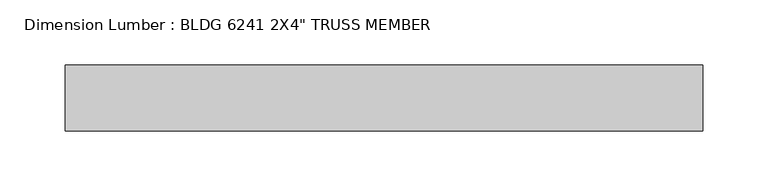
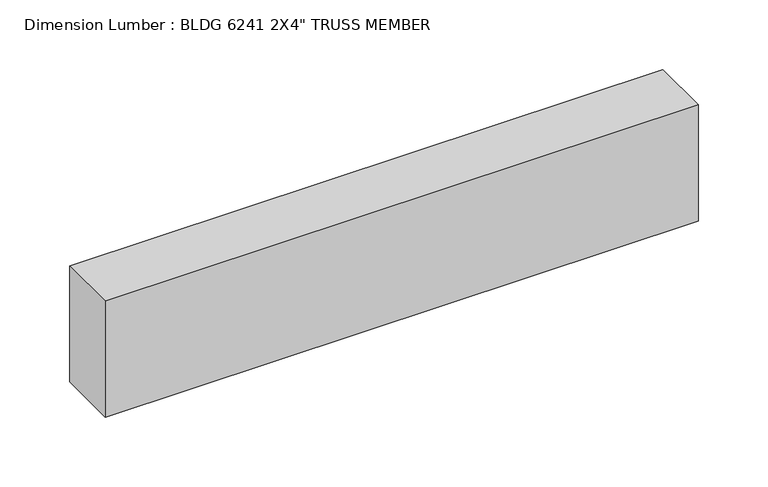
"""IFC4 building model written with IfcOpenShell, lengths in millimetres: beam geometry."""

from ifc_helpers import new_model, si_unit, frame, origin, place, context, project, spatial, polyline, outline, extrude, source, transform, mapped, element, save


def beam_7b8fa6d1(model_context):
    return source(origin(), model_context, "Body", "SweptSolid", [
        extrude(outline(polyline([(270.7395597, 25.4), (270.7395597, -25.4), (-219.9395597, -25.4), (-219.9395597, 25.4), (270.7395597, 25.4)])), frame((0.0, 0.0, -50.8), z_axis=(0.0, 0.0, 1.0), x_axis=(1.0, 0.0, 0.0)), (0.0, 0.0, 1.0), 101.6),
    ])


if __name__ == "__main__":
    model = new_model("IFC4")
    model_context = context("Model", 3, world=origin())
    ifc_project = project(units=[si_unit("LENGTHUNIT", "METRE", prefix="MILLI")], contexts=[model_context])
    site = spatial("IfcSite", under=ifc_project)
    building = spatial("IfcBuilding", under=site)
    placement = place(None, origin())
    beam_shape = beam_7b8fa6d1(model_context)
    element("IfcBeam", 1, ObjectType="Dimension Lumber : BLDG 6241 2X4\" TRUSS MEMBER", at=placement, inside=building, context=model_context, shape_type="MappedRepresentation", body=[
        mapped(beam_shape, transform((0.0, 0.0, 0.0), x_axis=(1.0, 0.0, 0.0), y_axis=(0.0, 1.0, 0.0), z_axis=(0.0, 0.0, 1.0))),
    ])
    save(model, "model.ifc")

# Revit data of these elements
# Type "Dimension Lumber : BLDG 6241 2X4\" TRUSS MEMBER"
#   Assembly Code = "B10"
#   A = 0.273472 SF
#   Length [instance default] = 5' - 0"
#   b = 0' - 2"
#   d = 0' - 4"
#   Structural Material [instance default] = Softwood, Lumber
# Element 1 (IfcBeam, "Dimension Lumber : BLDG 6241 2X4\" TRUSS MEMBER")
#   Materials on its faces: "Softwood, Lumber"
# Materials
#   "Softwood, Lumber": class "Wood", colour RGB 223 192 134, transparency 0, Description = "Pinus Echinata", Cost = 0
